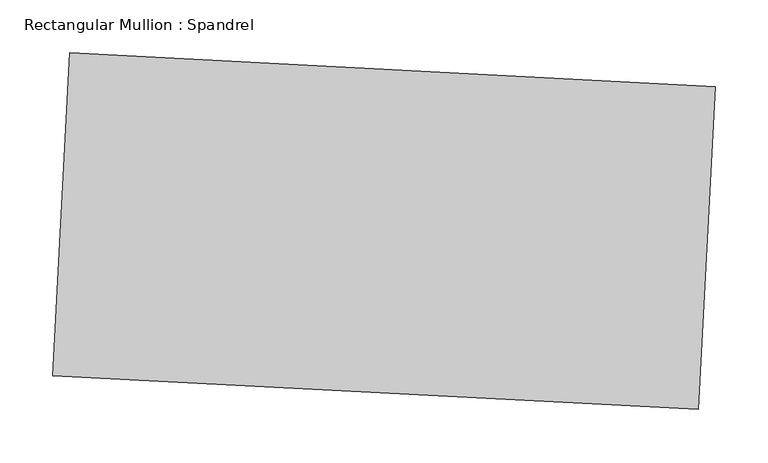
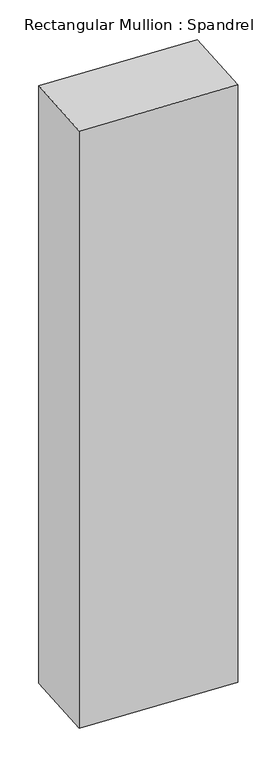
"""IFC4 building model written with IfcOpenShell, lengths in millimetres: member geometry, Rectangular Mullion : Spandrel."""

import ifcopenshell
import ifcopenshell.guid

model = None  # the IFC model being written
_history = None  # IfcOwnerHistory: only IFC2X3 demands one
_inside = {}  # id of a spatial element -> (the spatial element, [elements in it])
_under = {}  # id of a project, library or spatial element -> (it, [spatial elements below it])
_declared = {}  # id of a project -> (the project, [libraries it declares])
_typed = {}  # id of a type object -> (the type object, [elements of that type])
_made_of = {}  # id of a material, layer set ... -> (it, [elements and type objects made of it])


def new_model(schema):
    """Start an empty IFC model of exactly this schema.

    Asked for "IFC4X3", IfcOpenShell would pick the latest addendum, in which some entities
    have other attributes; the version numbers below select the first issue.
    IFC2X3 requires an IfcOwnerHistory on every rooted entity: one is made here for all.
    """
    global model, _history
    if schema == "IFC4X3":
        model = ifcopenshell.file(schema_version=(4, 3, 0, 0))
    else:
        model = ifcopenshell.file(schema=schema)
    _inside.clear()
    _under.clear()
    _declared.clear()
    _typed.clear()
    _made_of.clear()
    _history = None
    if model.schema == "IFC2X3":
        org = make("IfcOrganization", Name="unknown")
        user = make(
            "IfcPersonAndOrganization",
            ThePerson=make("IfcPerson", FamilyName="unknown"),
            TheOrganization=org,
        )
        app = make(
            "IfcApplication",
            ApplicationDeveloper=org,
            Version="unknown",
            ApplicationFullName="unknown",
            ApplicationIdentifier="unknown",
        )
        _history = make(
            "IfcOwnerHistory",
            OwningUser=user,
            OwningApplication=app,
            ChangeAction="ADDED",
            CreationDate=0,
        )
    return model


def make(cls, **values):
    """One entity of the class cls with the attributes given. An attribute that is None is left unset."""
    return model.create_entity(
        cls, **{name: value for name, value in values.items() if value is not None}
    )


def rooted(cls, **values):
    """An entity with a GlobalId (a new one), such as an element, a storey or a relation."""
    return make(cls, GlobalId=ifcopenshell.guid.new(), OwnerHistory=_history, **values)


def si_unit(unit_type, name, prefix=None):
    """IfcSIUnit, for example si_unit("LENGTHUNIT", "METRE", prefix="MILLI")."""
    return make("IfcSIUnit", UnitType=unit_type, Prefix=prefix, Name=name)


def assignment(units):
    """IfcUnitAssignment: the units of a project."""
    return None if units is None else make("IfcUnitAssignment", Units=units)


def point(xyz):
    """IfcCartesianPoint."""
    return None if xyz is None else make("IfcCartesianPoint", Coordinates=xyz)


def direction(xyz):
    """IfcDirection."""
    return None if xyz is None else make("IfcDirection", DirectionRatios=xyz)


def frame(location, z_axis=None, x_axis=None):
    """IfcAxis2Placement3D, a coordinate frame: its origin and axes. An axis left out is left unset."""
    return make(
        "IfcAxis2Placement3D",
        Location=point(location),
        Axis=direction(z_axis),
        RefDirection=direction(x_axis),
    )


def origin():
    """The frame at (0, 0, 0) with its axes left unset."""
    return frame((0.0, 0.0, 0.0))


def place(relative_to, where):
    """IfcLocalPlacement: puts the frame where relative to a parent placement (None: the world)."""
    return make(
        "IfcLocalPlacement", PlacementRelTo=relative_to, RelativePlacement=where
    )


def context(
    kind, dimensions, precision=None, world=None, true_north=None, identifier=None
):
    """IfcGeometricRepresentationContext, for example the 3D "Model" context."""
    return make(
        "IfcGeometricRepresentationContext",
        ContextIdentifier=identifier,
        ContextType=kind,
        CoordinateSpaceDimension=dimensions,
        Precision=precision,
        WorldCoordinateSystem=world,
        TrueNorth=true_north,
    )


def project(units=None, contexts=None):
    """IfcProject with its units and contexts."""
    return rooted(
        "IfcProject",
        Name="project",
        RepresentationContexts=contexts,
        UnitsInContext=assignment(units),
    )


def spatial(cls, under=None, at=None, **own):
    """A site, building, storey or space (cls), placed at a placement, below another one or the project."""
    s = rooted(cls, ObjectPlacement=at, **own)
    if under is not None:
        _under.setdefault(under.id(), (under, []))[1].append(s)
    return s


def polyline(points):
    """IfcPolyline through the points."""
    return make("IfcPolyline", Points=[point(p) for p in points])


def outline(outer, holes=None, kind="AREA"):
    """IfcArbitraryClosedProfileDef: a profile drawn as a closed curve; with holes, ...WithVoids."""
    if holes is None:
        return make("IfcArbitraryClosedProfileDef", ProfileType=kind, OuterCurve=outer)
    return make(
        "IfcArbitraryProfileDefWithVoids",
        ProfileType=kind,
        OuterCurve=outer,
        InnerCurves=holes,
    )


def extrude(swept, where, along, depth):
    """IfcExtrudedAreaSolid: the profile swept, set in the frame where, extruded along a direction by depth."""
    return make(
        "IfcExtrudedAreaSolid",
        SweptArea=swept,
        Position=where,
        ExtrudedDirection=direction(along),
        Depth=depth,
    )


def shape(context_of_items, identifier, shape_type, items):
    """IfcShapeRepresentation: the items that make up one representation, for example the "Body"."""
    return make(
        "IfcShapeRepresentation",
        ContextOfItems=context_of_items,
        RepresentationIdentifier=identifier,
        RepresentationType=shape_type,
        Items=items,
    )


def source(mapping_origin, context_of_items, identifier, shape_type, items):
    """IfcRepresentationMap: a shape defined once, which mapped items show again and again."""
    return make(
        "IfcRepresentationMap",
        MappingOrigin=mapping_origin,
        MappedRepresentation=shape(context_of_items, identifier, shape_type, items),
    )


def transform(
    local_origin,
    x_axis=None,
    y_axis=None,
    z_axis=None,
    scale=None,
    scale2=None,
    scale3=None,
    uniform=True,
):
    """IfcCartesianTransformationOperator3D, or its non-uniform kind. x_axis, y_axis, z_axis: its Axis1, 2, 3."""
    if uniform:
        return make(
            "IfcCartesianTransformationOperator3D",
            Axis1=direction(x_axis),
            Axis2=direction(y_axis),
            LocalOrigin=point(local_origin),
            Scale=scale,
            Axis3=direction(z_axis),
        )
    return make(
        "IfcCartesianTransformationOperator3DnonUniform",
        Axis1=direction(x_axis),
        Axis2=direction(y_axis),
        LocalOrigin=point(local_origin),
        Scale=scale,
        Axis3=direction(z_axis),
        Scale2=scale2,
        Scale3=scale3,
    )


def mapped(mapping_source, mapping_target):
    """IfcMappedItem: shows the shape of a source again, moved by a transform."""
    return make(
        "IfcMappedItem", MappingSource=mapping_source, MappingTarget=mapping_target
    )


def made_of(thing, what):
    """Note that an element or type object is made of a material, layer set ...; save() writes the relation."""
    if what is not None:
        _made_of.setdefault(what.id(), (what, []))[1].append(thing)
    return thing


def element(
    cls,
    number,
    at=None,
    inside=None,
    cuts=None,
    type_object=None,
    material=None,
    context=None,
    identifier="Body",
    shape_type=None,
    held_by="IfcProductDefinitionShape",
    body=None,
    shapes=None,
    **own,
):
    """One element of the class cls, such as IfcWall. Its Tag is "e" and its number.

    at: its placement. inside: the storey or other place that contains it. cuts: it is an
    opening in that element (IfcRelVoidsElement). A single representation is given by context,
    identifier, shape_type and body (its items); several are given by shapes. held_by: the class
    of the entity that holds the representations. save() writes the other relations.
    """
    e = rooted(cls, Tag="e%d" % number, ObjectPlacement=at, **own)
    if body is not None:
        shapes = [shape(context, identifier, shape_type, body)]
    if shapes is not None:
        e.Representation = make(held_by, Representations=shapes)
    if inside is not None:
        _inside.setdefault(inside.id(), (inside, []))[1].append(e)
    if cuts is not None:
        rooted(
            "IfcRelVoidsElement", RelatingBuildingElement=cuts, RelatedOpeningElement=e
        )
    if type_object is not None:
        _typed.setdefault(type_object.id(), (type_object, []))[1].append(e)
    return made_of(e, material)


def aggregate(whole, parts):
    """IfcRelAggregates: a whole, such as a stair, and the parts it consists of."""
    return rooted("IfcRelAggregates", RelatingObject=whole, RelatedObjects=parts)


def save(model, path):
    """Write the relations noted so far, then the file.

    IfcRelAggregates (storeys below a building ...), IfcRelContainedInSpatialStructure (elements
    in a storey), IfcRelDefinesByType, IfcRelAssociatesMaterial and IfcRelDeclares: one each for
    every whole, place, type object, material and project.
    """
    for whole, parts in _under.values():
        aggregate(whole, parts)
    for where, things in _inside.values():
        rooted(
            "IfcRelContainedInSpatialStructure",
            RelatedElements=things,
            RelatingStructure=where,
        )
    for kind, things in _typed.values():
        rooted("IfcRelDefinesByType", RelatedObjects=things, RelatingType=kind)
    for what, things in _made_of.values():
        rooted("IfcRelAssociatesMaterial", RelatedObjects=things, RelatingMaterial=what)
    for by, libraries in _declared.values():
        rooted("IfcRelDeclares", RelatingContext=by, RelatedDefinitions=libraries)
    model.write(path)


def rectangular_mullion_spandrel_52f45183(model_context):
    return source(origin(), model_context, "Body", "SweptSolid", [
        extrude(outline(polyline([(312.3582819, 136.2391416), (296.4062825, -168.1431406), (-312.3582819, -136.2391416), (-296.4062825, 168.1431406), (312.3582819, 136.2391416)])), frame((0.0, 0.0, -2501.3782228), z_axis=(0.0, 0.0, 1.0), x_axis=(1.0, 0.0, 0.0)), (0.0, 0.0, 1.0), 2501.3782228),
    ])


if __name__ == "__main__":
    model = new_model("IFC4")
    model_context = context("Model", 3, world=origin())
    ifc_project = project(units=[si_unit("LENGTHUNIT", "METRE", prefix="MILLI")], contexts=[model_context])
    site = spatial("IfcSite", under=ifc_project)
    building = spatial("IfcBuilding", under=site)
    placement = place(None, origin())
    rectangular_mullion_spandrel_shape = rectangular_mullion_spandrel_52f45183(model_context)
    element("IfcMember", 1, ObjectType="Rectangular Mullion : Spandrel", at=placement, inside=building, context=model_context, shape_type="MappedRepresentation", body=[
        mapped(rectangular_mullion_spandrel_shape, transform((0.0, 0.0, 0.0), x_axis=(1.0, 0.0, 0.0), y_axis=(0.0, 1.0, 0.0), z_axis=(0.0, 0.0, 1.0))),
    ])
    save(model, "model.ifc")

# Revit data of these elements
# Type "Rectangular Mullion : Spandrel"
#   built-in parameter 1007304 = 1 (stored number, unit not read)
#   built-in parameter 1007301 = 1 (stored number, unit not read)
#   built-in parameter 1007300 = 1 (stored number, unit not read)
# Element 1 (IfcMember, "Rectangular Mullion : Spandrel")
#   Materials on its faces: "Aluminum"
# Materials
#   "Aluminum": class "Metal", colour RGB 247 247 247, transparency 0, Description = "Aluminum 6061", Cost = 0
